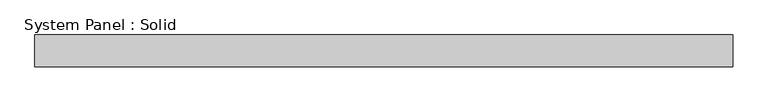
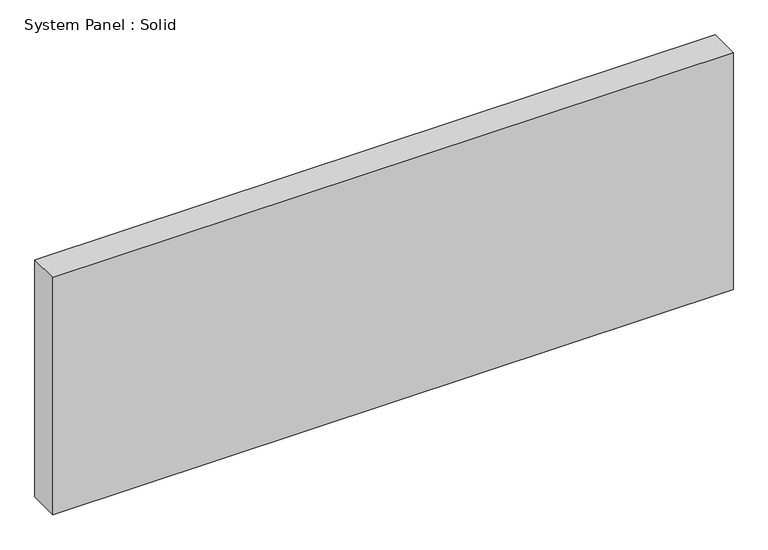
"""IFC4 building model written with IfcOpenShell, lengths in millimetres: plate geometry, System Panel : Solid."""

from ifc_helpers import new_model, si_unit, origin, origin_with_axes, place, context, project, spatial, polyline, outline, extrude, source, transform, mapped, element, save


def system_panel_solid_037144dd(model_context):
    return source(origin(), model_context, "Body", "SweptSolid", [
        extrude(outline(polyline([(697.4416668, -44.45), (-697.4416668, -44.45), (-697.4416668, 19.05), (697.4416668, 19.05), (697.4416668, -44.45)])), origin_with_axes(), (0.0, 0.0, 1.0), 514.35),
    ])


if __name__ == "__main__":
    model = new_model("IFC4")
    model_context = context("Model", 3, world=origin())
    ifc_project = project(units=[si_unit("LENGTHUNIT", "METRE", prefix="MILLI")], contexts=[model_context])
    site = spatial("IfcSite", under=ifc_project)
    building = spatial("IfcBuilding", under=site)
    placement = place(None, origin())
    system_panel_solid_shape = system_panel_solid_037144dd(model_context)
    element("IfcPlate", 1, ObjectType="System Panel : Solid", at=placement, inside=building, context=model_context, shape_type="MappedRepresentation", body=[
        mapped(system_panel_solid_shape, transform((0.0, 0.0, 0.0), x_axis=(1.0, 0.0, 0.0), y_axis=(0.0, 1.0, 0.0), z_axis=(0.0, 0.0, 1.0))),
    ])
    save(model, "model.ifc")

# Revit data of these elements
# Type "System Panel : Solid"
#   Construction Type Id = "MDOOR"
#   Analytic Construction = "Metal"
#   Visual Light Transmittance = 0
#   Solar Heat Gain Coefficient = 0
#   Heat Transfer Coefficient (U) = 0.651978 BTU/(h·ft²·°F)
#   Define Thermal Properties by = 1
# Element 1 (IfcPlate, "System Panel : Solid")
#   Materials on its faces: "Default"
# Materials
#   "Default": class "Miscellaneous", colour RGB 127 127 127, transparency 0, Cost = 0
